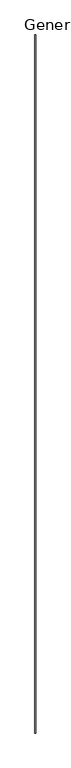
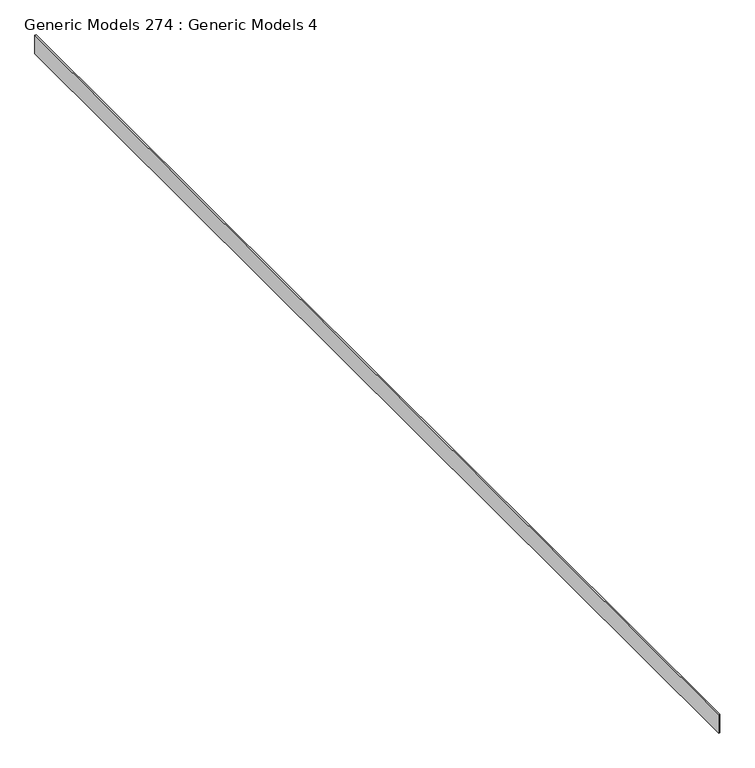
"""IFC4 building model written with IfcOpenShell, lengths in millimetres: proxy geometry, Generic Models 274 : Generic Models 4."""

from ifc_helpers import new_model, si_unit, frame, origin, place, context, project, spatial, polyline, outline, extrude, source, transform, mapped, element, save


def generic_models_274_generic_models_4_82473f9f(model_context):
    return source(origin(), model_context, "Body", "SweptSolid", [
        extrude(outline(polyline([(7253.8514146, -6864.9230338), (7234.8014146, -6864.9230338), (7234.8014146, 11778.6769662), (7253.8514146, 11778.6769662), (7253.8514146, -6864.9230338)])), frame((0.0, 0.0, 126809.341198), z_axis=(0.0, 0.0, 1.0), x_axis=(1.0, 0.0, 0.0)), (0.0, 0.0, 1.0), 307.5954552),
    ])


if __name__ == "__main__":
    model = new_model("IFC4")
    model_context = context("Model", 3, world=origin())
    ifc_project = project(units=[si_unit("LENGTHUNIT", "METRE", prefix="MILLI")], contexts=[model_context])
    site = spatial("IfcSite", under=ifc_project)
    building = spatial("IfcBuilding", under=site)
    placement = place(None, origin())
    generic_models_274_generic_models_4_shape = generic_models_274_generic_models_4_82473f9f(model_context)
    element("IfcBuildingElementProxy", 1, Name="Generic Models 274 : Generic Models 4", ObjectType="Generic Models 274 : Generic Models 4", at=placement, inside=building, context=model_context, shape_type="MappedRepresentation", body=[
        mapped(generic_models_274_generic_models_4_shape, transform((0.0, 0.0, 0.0), x_axis=(1.0, 0.0, 0.0), y_axis=(0.0, 1.0, 0.0), z_axis=(0.0, 0.0, 1.0))),
    ])
    save(model, "model.ifc")

# Revit data of these elements
# Element 1 (IfcBuildingElementProxy, "Generic Models 274 : Generic Models 4")
#   Materials on its faces: "_CDX PLYWOOD - SEE STRUCT DWGs"
# Materials
#   "_CDX PLYWOOD - SEE STRUCT DWGs": class "Generic", colour RGB 98 75 74, transparency 0, Cost = 0
